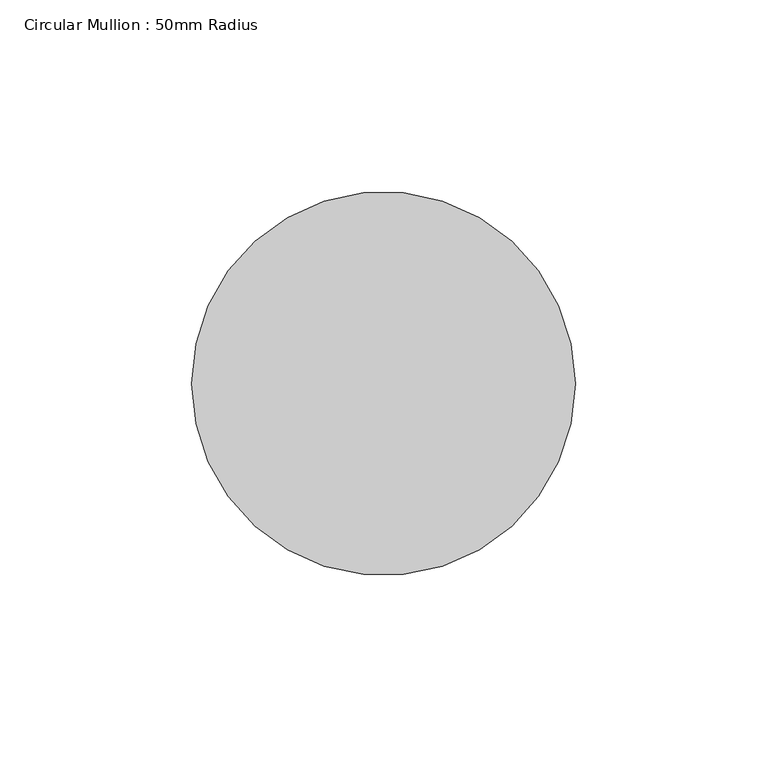
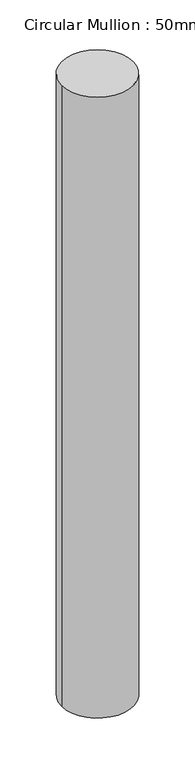
"""IFC4 building model written with IfcOpenShell, lengths in millimetres: member geometry, Circular Mullion : 50mm Radius."""

from ifc_helpers import new_model, si_unit, point, frame, origin, origin_2d, place, context, project, spatial, circle_curve, trimmed, segment, composite_curve, outline, extrude, source, transform, mapped, element, save


def circular_mullion_50mm_radius_c5039d41(model_context):
    return source(origin(), model_context, "Body", "SweptSolid", [
        extrude(outline(composite_curve([segment(trimmed(circle_curve(origin_2d(), 50.0), [point((50.0, 0.0))], [point((-50.0, 0.0))], False, "CARTESIAN"), True, "CONTINUOUS"), segment(trimmed(circle_curve(origin_2d(), 50.0), [point((-50.0, 0.0))], [point((50.0, 0.0))], False, "CARTESIAN"), True, "CONTINUOUS")], self_intersect=False)), frame((0.0, 0.0, -920.6582589), z_axis=(0.0, 0.0, 1.0), x_axis=(1.0, 0.0, 0.0)), (0.0, 0.0, 1.0), 920.6582589),
    ])


if __name__ == "__main__":
    model = new_model("IFC4")
    model_context = context("Model", 3, world=origin())
    ifc_project = project(units=[si_unit("LENGTHUNIT", "METRE", prefix="MILLI")], contexts=[model_context])
    site = spatial("IfcSite", under=ifc_project)
    building = spatial("IfcBuilding", under=site)
    placement = place(None, origin())
    circular_mullion_50mm_radius_shape = circular_mullion_50mm_radius_c5039d41(model_context)
    element("IfcMember", 1, ObjectType="Circular Mullion : 50mm Radius", at=placement, inside=building, context=model_context, shape_type="MappedRepresentation", body=[
        mapped(circular_mullion_50mm_radius_shape, transform((0.0, 0.0, 0.0), x_axis=(1.0, 0.0, 0.0), y_axis=(0.0, 1.0, 0.0), z_axis=(0.0, 0.0, 1.0))),
    ])
    save(model, "model.ifc")

# Revit data of these elements
# Type "Circular Mullion : 50mm Radius"
#   built-in parameter 1007350 = 0.164042 (stored number, unit not read)
# Element 1 (IfcMember, "Circular Mullion : 50mm Radius")
#   Materials on its faces: "Aluminium"
# Materials
#   "Aluminium": class "Metal", colour RGB 247 247 247, transparency 0, Description = "Aluminium 6061", Cost = 0
